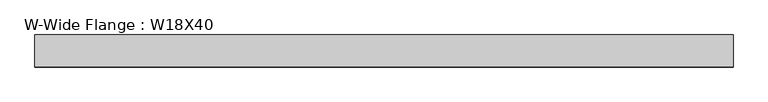
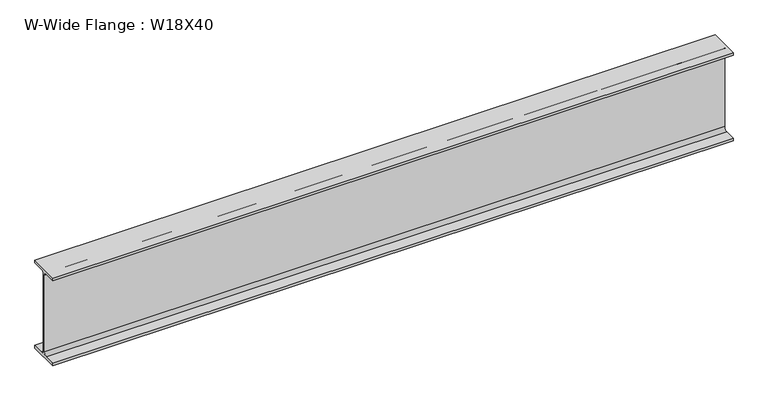
"""IFC4 building model written with IfcOpenShell, lengths in millimetres: beam geometry, W-Wide Flange : W18X40."""

from ifc_helpers import new_model, si_unit, point, frame, frame_2d, origin, place, context, project, spatial, polyline, circle_curve, trimmed, segment, composite_curve, outline, extrude, source, transform, mapped, element, save


def w_wide_flange_w18x40_ed8c275d(model_context):
    return source(origin(), model_context, "Body", "SweptSolid", [
        extrude(outline(composite_curve([segment(polyline([(76.454, -213.995), (76.454, -227.33), (-76.454, -227.33), (-76.454, -213.995), (-20.828, -213.995)]), True, "CONTINUOUS"), segment(trimmed(circle_curve(frame_2d((-20.828, -197.1675)), 16.8275), [point((-20.828, -213.995))], [point((-4.0005, -197.1675))], True, "CARTESIAN"), True, "CONTINUOUS"), segment(polyline([(-4.0005, -197.1675), (-4.0005, 197.1675)]), True, "CONTINUOUS"), segment(trimmed(circle_curve(frame_2d((-20.828, 197.1675)), 16.8275), [point((-4.0005, 197.1675))], [point((-20.828, 213.995))], True, "CARTESIAN"), True, "CONTINUOUS"), segment(polyline([(-20.828, 213.995), (-76.454, 213.995), (-76.454, 227.33), (76.454, 227.33), (76.454, 213.995), (20.828, 213.995)]), True, "CONTINUOUS"), segment(trimmed(circle_curve(frame_2d((20.828, 197.1675)), 16.8275), [point((20.828, 213.995))], [point((4.0005, 197.1675))], True, "CARTESIAN"), True, "CONTINUOUS"), segment(polyline([(4.0005, 197.1675), (4.0005, -197.1675)]), True, "CONTINUOUS"), segment(trimmed(circle_curve(frame_2d((20.828, -197.1675)), 16.8275), [point((4.0005, -197.1675))], [point((20.828, -213.995))], True, "CARTESIAN"), True, "CONTINUOUS"), segment(polyline([(20.828, -213.995), (76.454, -213.995)]), True, "CONTINUOUS")], self_intersect=False)), frame((-1701.7999994, 0.0, 0.0), z_axis=(1.0, 0.0, 0.0), x_axis=(0.0, 1.0, 0.0)), (0.0, 0.0, 1.0), 3327.3999994),
    ])


if __name__ == "__main__":
    model = new_model("IFC4")
    model_context = context("Model", 3, world=origin())
    ifc_project = project(units=[si_unit("LENGTHUNIT", "METRE", prefix="MILLI")], contexts=[model_context])
    site = spatial("IfcSite", under=ifc_project)
    building = spatial("IfcBuilding", under=site)
    placement = place(None, origin())
    w_wide_flange_w18x40_shape = w_wide_flange_w18x40_ed8c275d(model_context)
    element("IfcBeam", 1, ObjectType="W-Wide Flange : W18X40", at=placement, inside=building, context=model_context, shape_type="MappedRepresentation", body=[
        mapped(w_wide_flange_w18x40_shape, transform((0.0, 0.0, 0.0), x_axis=(1.0, 0.0, 0.0), y_axis=(0.0, 1.0, 0.0), z_axis=(0.0, 0.0, 1.0))),
    ])
    save(model, "model.ifc")

# Revit data of these elements
# Type "W-Wide Flange : W18X40"
#   Assembly Code = "B10"
#   W = 40
#   Length [instance default] = 5' - 0"
#   bf = 0' - 6.02"
#   d = 1' - 5.9"
#   k = 0' - 1 3/16"
#   k2 = 0' - 0.6625"
#   tf = 0' - 0.525"
#   tw = 0' - 0.315"
#   A = 0.0819444 SF
#   Structural Material [instance default] = Steel ASTM A992
# Element 1 (IfcBeam, "W-Wide Flange : W18X40")
#   Materials on its faces: "Steel ASTM A992"
# Materials
#   "Steel ASTM A992": class "Metal", colour RGB 199 199 199, transparency 0, Description = "Structural steel 50ksi", Cost = 0
